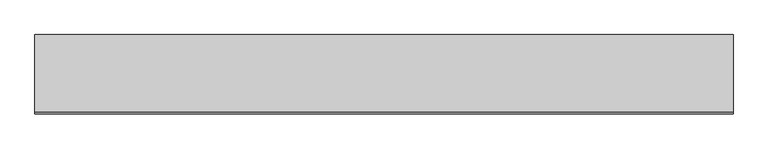
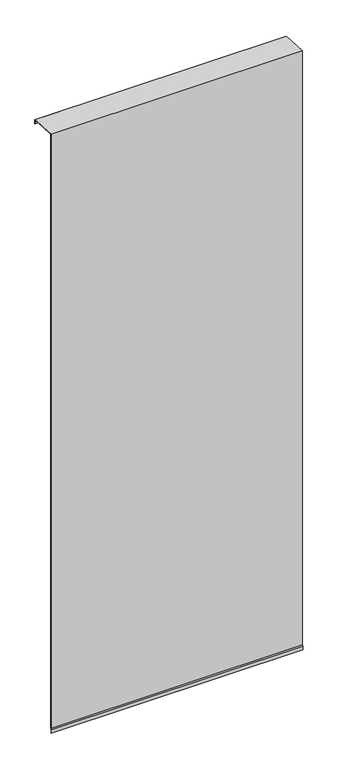
"""IFC4 building model written with IfcOpenShell, lengths in millimetres: proxy geometry, Generic Models 7:Generic Models 1:5:Generic Models 1:5 : Generic Models 7:Generic Models 1:337419:5 : Generic Models 7:Generic Models 1:5:Generic Models 1:5 : Generic Models 7:Generic Models 1:337419:311462."""

from ifc_helpers import new_model, si_unit, frame, origin, place, context, project, spatial, polyline, outline, extrude, source, transform, mapped, element, save


def generic_models_4a7ecb1e(model_context):
    return source(origin(), model_context, "Body", "SweptSolid", [
        extrude(outline(polyline([(-579045.2451279, 84.8477111), (-579051.2612667, 76.2557745), (-579051.2612667, 40.0253703), (-579052.8487667, 40.0253703), (-579052.8487667, 76.7563114), (-579046.8326279, 85.348248), (-579046.8326279, 6180.7780819), (-578776.0601341, 6166.5874968), (-578776.0601341, 6125.115987), (-578777.6476341, 6125.115987), (-578777.6476341, 6165.0810156), (-579045.2451279, 6179.105206), (-579045.2451279, 84.8477111)])), frame((570452.6367239, 0.0, 0.0), z_axis=(1.0, 0.0, 0.0), x_axis=(0.0, 1.0, 0.0)), (0.0, 0.0, 1.0), 2444.75),
    ])


if __name__ == "__main__":
    model = new_model("IFC4")
    model_context = context("Model", 3, world=origin())
    ifc_project = project(units=[si_unit("LENGTHUNIT", "METRE", prefix="MILLI")], contexts=[model_context])
    site = spatial("IfcSite", under=ifc_project)
    building = spatial("IfcBuilding", under=site)
    placement = place(None, origin())
    generic_models_shape = generic_models_4a7ecb1e(model_context)
    element("IfcBuildingElementProxy", 1, Name="Generic Models 7:Generic Models 1:5:Generic Models 1:5 : Generic Models 7:Generic Models 1:337419:5 : Generic Models 7:Generic Models 1:5:Generic Models 1:5 : Generic Models 7:Generic Models 1:337419:311462", ObjectType="Generic Models 7:Generic Models 1:5:Generic Models 1:5 : Generic Models 7:Generic Models 1:337419:5 : Generic Models 7:Generic Models 1:5:Generic Models 1:5 : Generic Models 7:Generic Models 1:337419:311462", at=placement, inside=building, context=model_context, shape_type="MappedRepresentation", body=[
        mapped(generic_models_shape, transform((0.0, 0.0, 0.0), x_axis=(1.0, 0.0, 0.0), y_axis=(0.0, 1.0, 0.0), z_axis=(0.0, 0.0, 1.0))),
    ])
    save(model, "model.ifc")

# Revit data of these elements
# Type "Generic Models 7:Generic Models 1:5:Generic Models 1:5 : Generic Models 7:Generic Models 1:337419:5 : Generic Models 7:Generic Models 1:5:Generic Models 1:5 : Generic Models 7:Generic Models 1:337419:311462"
#   NameOverride = "Generic Models 7:Generic Models 1:5:Generic Models 1:5 : Generic Models 7:Generic Models 1:337419:311462"
#   ObjectTypeOverride = "Generic Models 1:5 : Generic Models 7:Generic Models 1:337419"
#   Reference = "Generic Models 1"
#   Tag = "311462"
# Element 1 (IfcBuildingElementProxy, "Generic Models 7:Generic Models 1:5:Generic Models 1:5 : Generic Models 7:Generic Models 1:337419:5 : Generic Models 7:Generic Models 1:5:Generic Models 1:5 : Generic Models 7:Generic Models 1:337419:311462")
#   Materials on its faces: "UV STABLE WATER RESISTANT VAPOR PERMEABLE AIR BARRIER"
# Materials
#   "UV STABLE WATER RESISTANT VAPOR PERMEABLE AIR BARRIER": class "Generic", colour RGB 51 162 45, transparency 0, Description = "Polyethylene film membrane", Cost = 0
